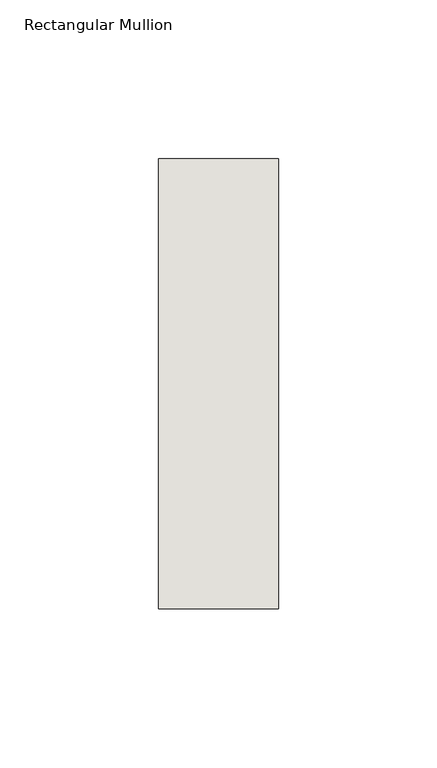
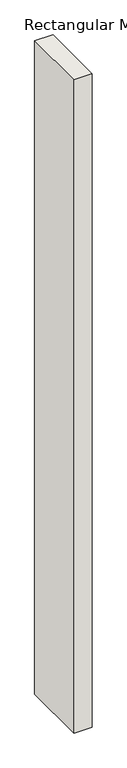
"""IFC4 building model written with IfcOpenShell, lengths in millimetres: wall geometry, Rectangular Mullion : NLRS_21_CWM_hsb-regel 38x142_gen_rsf."""

from ifc_helpers import new_model, si_unit, frame, origin, place, context, project, spatial, polyline, outline, extrude, source, transform, mapped, element, save


def rectangular_mullion_dc0a3d83(model_context):
    return source(origin(), model_context, "Body", "SweptSolid", [
        extrude(outline(polyline([(-38.0, -71.0), (-38.0, 71.0), (0.0, 71.0), (0.0, -71.0), (-38.0, -71.0)])), frame((0.0, 0.0, -1440.0), z_axis=(0.0, 0.0, 1.0), x_axis=(1.0, 0.0, 0.0)), (0.0, 0.0, 1.0), 1440.0),
    ])


if __name__ == "__main__":
    model = new_model("IFC4")
    model_context = context("Model", 3, world=origin())
    ifc_project = project(units=[si_unit("LENGTHUNIT", "METRE", prefix="MILLI")], contexts=[model_context])
    site = spatial("IfcSite", under=ifc_project)
    building = spatial("IfcBuilding", under=site)
    placement = place(None, origin())
    rectangular_mullion_shape = rectangular_mullion_dc0a3d83(model_context)
    element("IfcWall", 1, ObjectType="Rectangular Mullion : NLRS_21_CWM_hsb-regel 38x142_gen_rsf", at=placement, inside=building, context=model_context, shape_type="MappedRepresentation", body=[
        mapped(rectangular_mullion_shape, transform((0.0, 0.0, 0.0), x_axis=(1.0, 0.0, 0.0), y_axis=(0.0, 1.0, 0.0), z_axis=(0.0, 0.0, 1.0))),
    ])
    save(model, "model.ifc")

# Revit data of these elements
# Type "Rectangular Mullion : NLRS_21_CWM_hsb-regel 38x142_gen_rsf"
#   Type IfcGUID = "07M7mRoiH1CR8m_RSKIwpF"
#   Assembly Code = "21.10"
#   IfcExportAs = "IfcWall"
#   built-in parameter 1007322 = 0.465879 (stored number, unit not read)
#   built-in parameter 1007321 = 0.062336 (stored number, unit not read)
#   built-in parameter 1007320 = 0.062336 (stored number, unit not read)
# Element 1 (IfcWall, "Rectangular Mullion : NLRS_21_CWM_hsb-regel 38x142_gen_rsf")
#   Materials on its faces: "NLRS_i2_hout naaldhout vuren_gen_rsf"
# Materials
#   "NLRS_i2_hout naaldhout vuren_gen_rsf": class "I - Hout", colour RGB 234 199 147, transparency 0, Keynote = "i2", Manufacturer = "Revit Standards Foundation", URL = "www.revitstandards.org", Description = "hout vuren", Cost = 0
